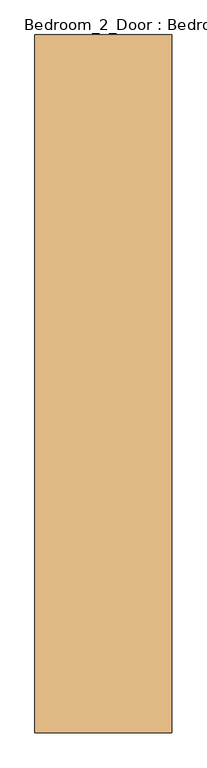
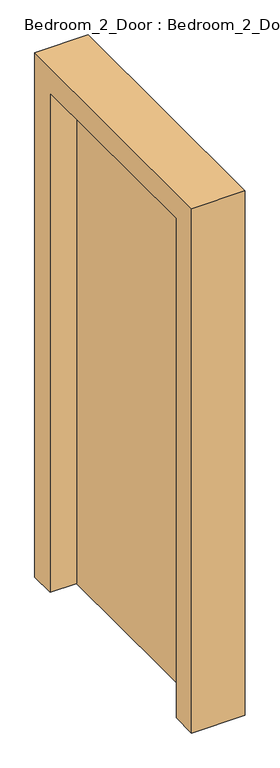
"""IFC4 building model written with IfcOpenShell, lengths in millimetres: door geometry, Bedroom_2_Door : Bedroom_2_Door."""

from ifc_helpers import new_model, si_unit, frame, origin, place, context, project, spatial, polyline, outline, extrude, source, transform, mapped, element, save


def bedroom_2_door_bedroom_2_door_3f2e3542(model_context):
    return source(origin(), model_context, "Body", "SweptSolid", [
        extrude(outline(polyline([(1565.0, 7875.0), (1565.0, 8695.0), (1665.0, 8695.0), (1665.0, 7875.0), (1565.0, 7875.0)])), frame((0.0, 0.0, 250.0), z_axis=(0.0, 0.0, 1.0), x_axis=(1.0, 0.0, 0.0)), (0.0, 0.0, 1.0), 1980.0),
        extrude(outline(polyline([(8795.0, 250.0), (8695.0, 250.0), (8695.0, 2230.0), (7875.0, 2230.0), (7875.0, 250.0), (7775.0, 250.0), (7775.0, 2330.0), (8795.0, 2330.0), (8795.0, 250.0)])), frame((1465.0, 0.0, 0.0), z_axis=(1.0, 0.0, 0.0), x_axis=(0.0, 1.0, 0.0)), (0.0, 0.0, 1.0), 200.0),
    ])


if __name__ == "__main__":
    model = new_model("IFC4")
    model_context = context("Model", 3, world=origin())
    ifc_project = project(units=[si_unit("LENGTHUNIT", "METRE", prefix="MILLI")], contexts=[model_context])
    site = spatial("IfcSite", under=ifc_project)
    building = spatial("IfcBuilding", under=site)
    placement = place(None, origin())
    bedroom_2_door_bedroom_2_door_shape = bedroom_2_door_bedroom_2_door_3f2e3542(model_context)
    element("IfcDoor", 1, ObjectType="Bedroom_2_Door : Bedroom_2_Door", at=placement, inside=building, context=model_context, shape_type="MappedRepresentation", body=[
        mapped(bedroom_2_door_bedroom_2_door_shape, transform((0.0, 0.0, 0.0), x_axis=(1.0, 0.0, 0.0), y_axis=(0.0, 1.0, 0.0), z_axis=(0.0, 0.0, 1.0))),
    ])
    save(model, "model.ifc")

# Revit data of these elements
# Type "Bedroom_2_Door : Bedroom_2_Door"
#   Type Mark = "49"
#   NameOverride = "Bedroom_2_Door"
# Element 1 (IfcDoor, "Bedroom_2_Door : Bedroom_2_Door")
#   Materials on its faces: "IfcSurfaceStyle #392"
# Materials
#   "IfcSurfaceStyle #392": class "Unassigned", colour RGB 204 204 204, transparency 0
